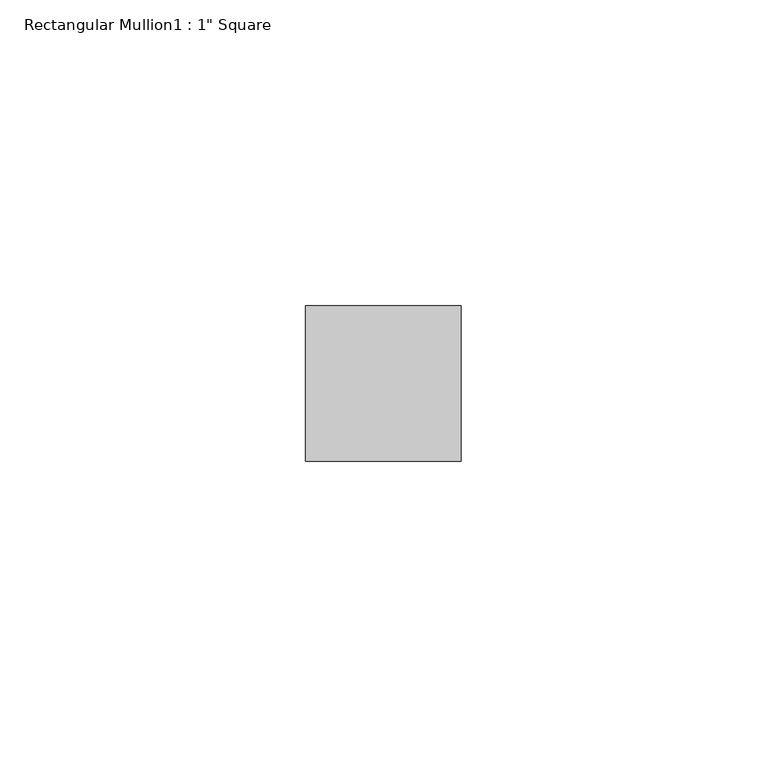
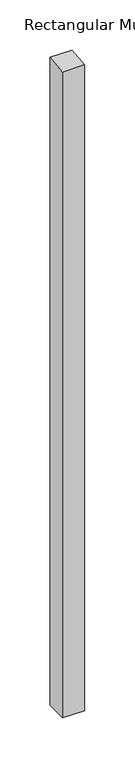
"""IFC4 building model written with IfcOpenShell, lengths in millimetres: member geometry."""

import ifcopenshell
import ifcopenshell.guid

model = None  # the IFC model being written
_history = None  # IfcOwnerHistory: only IFC2X3 demands one
_inside = {}  # id of a spatial element -> (the spatial element, [elements in it])
_under = {}  # id of a project, library or spatial element -> (it, [spatial elements below it])
_declared = {}  # id of a project -> (the project, [libraries it declares])
_typed = {}  # id of a type object -> (the type object, [elements of that type])
_made_of = {}  # id of a material, layer set ... -> (it, [elements and type objects made of it])


def new_model(schema):
    """Start an empty IFC model of exactly this schema.

    Asked for "IFC4X3", IfcOpenShell would pick the latest addendum, in which some entities
    have other attributes; the version numbers below select the first issue.
    IFC2X3 requires an IfcOwnerHistory on every rooted entity: one is made here for all.
    """
    global model, _history
    if schema == "IFC4X3":
        model = ifcopenshell.file(schema_version=(4, 3, 0, 0))
    else:
        model = ifcopenshell.file(schema=schema)
    _inside.clear()
    _under.clear()
    _declared.clear()
    _typed.clear()
    _made_of.clear()
    _history = None
    if model.schema == "IFC2X3":
        org = make("IfcOrganization", Name="unknown")
        user = make(
            "IfcPersonAndOrganization",
            ThePerson=make("IfcPerson", FamilyName="unknown"),
            TheOrganization=org,
        )
        app = make(
            "IfcApplication",
            ApplicationDeveloper=org,
            Version="unknown",
            ApplicationFullName="unknown",
            ApplicationIdentifier="unknown",
        )
        _history = make(
            "IfcOwnerHistory",
            OwningUser=user,
            OwningApplication=app,
            ChangeAction="ADDED",
            CreationDate=0,
        )
    return model


def make(cls, **values):
    """One entity of the class cls with the attributes given. An attribute that is None is left unset."""
    return model.create_entity(
        cls, **{name: value for name, value in values.items() if value is not None}
    )


def rooted(cls, **values):
    """An entity with a GlobalId (a new one), such as an element, a storey or a relation."""
    return make(cls, GlobalId=ifcopenshell.guid.new(), OwnerHistory=_history, **values)


def si_unit(unit_type, name, prefix=None):
    """IfcSIUnit, for example si_unit("LENGTHUNIT", "METRE", prefix="MILLI")."""
    return make("IfcSIUnit", UnitType=unit_type, Prefix=prefix, Name=name)


def assignment(units):
    """IfcUnitAssignment: the units of a project."""
    return None if units is None else make("IfcUnitAssignment", Units=units)


def point(xyz):
    """IfcCartesianPoint."""
    return None if xyz is None else make("IfcCartesianPoint", Coordinates=xyz)


def direction(xyz):
    """IfcDirection."""
    return None if xyz is None else make("IfcDirection", DirectionRatios=xyz)


def frame(location, z_axis=None, x_axis=None):
    """IfcAxis2Placement3D, a coordinate frame: its origin and axes. An axis left out is left unset."""
    return make(
        "IfcAxis2Placement3D",
        Location=point(location),
        Axis=direction(z_axis),
        RefDirection=direction(x_axis),
    )


def origin():
    """The frame at (0, 0, 0) with its axes left unset."""
    return frame((0.0, 0.0, 0.0))


def place(relative_to, where):
    """IfcLocalPlacement: puts the frame where relative to a parent placement (None: the world)."""
    return make(
        "IfcLocalPlacement", PlacementRelTo=relative_to, RelativePlacement=where
    )


def context(
    kind, dimensions, precision=None, world=None, true_north=None, identifier=None
):
    """IfcGeometricRepresentationContext, for example the 3D "Model" context."""
    return make(
        "IfcGeometricRepresentationContext",
        ContextIdentifier=identifier,
        ContextType=kind,
        CoordinateSpaceDimension=dimensions,
        Precision=precision,
        WorldCoordinateSystem=world,
        TrueNorth=true_north,
    )


def project(units=None, contexts=None):
    """IfcProject with its units and contexts."""
    return rooted(
        "IfcProject",
        Name="project",
        RepresentationContexts=contexts,
        UnitsInContext=assignment(units),
    )


def spatial(cls, under=None, at=None, **own):
    """A site, building, storey or space (cls), placed at a placement, below another one or the project."""
    s = rooted(cls, ObjectPlacement=at, **own)
    if under is not None:
        _under.setdefault(under.id(), (under, []))[1].append(s)
    return s


def polyline(points):
    """IfcPolyline through the points."""
    return make("IfcPolyline", Points=[point(p) for p in points])


def outline(outer, holes=None, kind="AREA"):
    """IfcArbitraryClosedProfileDef: a profile drawn as a closed curve; with holes, ...WithVoids."""
    if holes is None:
        return make("IfcArbitraryClosedProfileDef", ProfileType=kind, OuterCurve=outer)
    return make(
        "IfcArbitraryProfileDefWithVoids",
        ProfileType=kind,
        OuterCurve=outer,
        InnerCurves=holes,
    )


def extrude(swept, where, along, depth):
    """IfcExtrudedAreaSolid: the profile swept, set in the frame where, extruded along a direction by depth."""
    return make(
        "IfcExtrudedAreaSolid",
        SweptArea=swept,
        Position=where,
        ExtrudedDirection=direction(along),
        Depth=depth,
    )


def shape(context_of_items, identifier, shape_type, items):
    """IfcShapeRepresentation: the items that make up one representation, for example the "Body"."""
    return make(
        "IfcShapeRepresentation",
        ContextOfItems=context_of_items,
        RepresentationIdentifier=identifier,
        RepresentationType=shape_type,
        Items=items,
    )


def source(mapping_origin, context_of_items, identifier, shape_type, items):
    """IfcRepresentationMap: a shape defined once, which mapped items show again and again."""
    return make(
        "IfcRepresentationMap",
        MappingOrigin=mapping_origin,
        MappedRepresentation=shape(context_of_items, identifier, shape_type, items),
    )


def transform(
    local_origin,
    x_axis=None,
    y_axis=None,
    z_axis=None,
    scale=None,
    scale2=None,
    scale3=None,
    uniform=True,
):
    """IfcCartesianTransformationOperator3D, or its non-uniform kind. x_axis, y_axis, z_axis: its Axis1, 2, 3."""
    if uniform:
        return make(
            "IfcCartesianTransformationOperator3D",
            Axis1=direction(x_axis),
            Axis2=direction(y_axis),
            LocalOrigin=point(local_origin),
            Scale=scale,
            Axis3=direction(z_axis),
        )
    return make(
        "IfcCartesianTransformationOperator3DnonUniform",
        Axis1=direction(x_axis),
        Axis2=direction(y_axis),
        LocalOrigin=point(local_origin),
        Scale=scale,
        Axis3=direction(z_axis),
        Scale2=scale2,
        Scale3=scale3,
    )


def mapped(mapping_source, mapping_target):
    """IfcMappedItem: shows the shape of a source again, moved by a transform."""
    return make(
        "IfcMappedItem", MappingSource=mapping_source, MappingTarget=mapping_target
    )


def made_of(thing, what):
    """Note that an element or type object is made of a material, layer set ...; save() writes the relation."""
    if what is not None:
        _made_of.setdefault(what.id(), (what, []))[1].append(thing)
    return thing


def element(
    cls,
    number,
    at=None,
    inside=None,
    cuts=None,
    type_object=None,
    material=None,
    context=None,
    identifier="Body",
    shape_type=None,
    held_by="IfcProductDefinitionShape",
    body=None,
    shapes=None,
    **own,
):
    """One element of the class cls, such as IfcWall. Its Tag is "e" and its number.

    at: its placement. inside: the storey or other place that contains it. cuts: it is an
    opening in that element (IfcRelVoidsElement). A single representation is given by context,
    identifier, shape_type and body (its items); several are given by shapes. held_by: the class
    of the entity that holds the representations. save() writes the other relations.
    """
    e = rooted(cls, Tag="e%d" % number, ObjectPlacement=at, **own)
    if body is not None:
        shapes = [shape(context, identifier, shape_type, body)]
    if shapes is not None:
        e.Representation = make(held_by, Representations=shapes)
    if inside is not None:
        _inside.setdefault(inside.id(), (inside, []))[1].append(e)
    if cuts is not None:
        rooted(
            "IfcRelVoidsElement", RelatingBuildingElement=cuts, RelatedOpeningElement=e
        )
    if type_object is not None:
        _typed.setdefault(type_object.id(), (type_object, []))[1].append(e)
    return made_of(e, material)


def aggregate(whole, parts):
    """IfcRelAggregates: a whole, such as a stair, and the parts it consists of."""
    return rooted("IfcRelAggregates", RelatingObject=whole, RelatedObjects=parts)


def save(model, path):
    """Write the relations noted so far, then the file.

    IfcRelAggregates (storeys below a building ...), IfcRelContainedInSpatialStructure (elements
    in a storey), IfcRelDefinesByType, IfcRelAssociatesMaterial and IfcRelDeclares: one each for
    every whole, place, type object, material and project.
    """
    for whole, parts in _under.values():
        aggregate(whole, parts)
    for where, things in _inside.values():
        rooted(
            "IfcRelContainedInSpatialStructure",
            RelatedElements=things,
            RelatingStructure=where,
        )
    for kind, things in _typed.values():
        rooted("IfcRelDefinesByType", RelatedObjects=things, RelatingType=kind)
    for what, things in _made_of.values():
        rooted("IfcRelAssociatesMaterial", RelatedObjects=things, RelatingMaterial=what)
    for by, libraries in _declared.values():
        rooted("IfcRelDeclares", RelatingContext=by, RelatedDefinitions=libraries)
    model.write(path)


def member_382b1cd2(model_context):
    return source(origin(), model_context, "Body", "SweptSolid", [
        extrude(outline(polyline([(-44.45, -4.2341647), (-19.05, -1.814642), (-19.05, -790.0272395), (-44.45, -790.0272395), (-44.45, -4.2341647)])), frame((-25.4, 0.0, 0.0), z_axis=(1.0, 0.0, 0.0), x_axis=(0.0, 1.0, 0.0)), (0.0, 0.0, 1.0), 25.4),
    ])


if __name__ == "__main__":
    model = new_model("IFC4")
    model_context = context("Model", 3, world=origin())
    ifc_project = project(units=[si_unit("LENGTHUNIT", "METRE", prefix="MILLI")], contexts=[model_context])
    site = spatial("IfcSite", under=ifc_project)
    building = spatial("IfcBuilding", under=site)
    placement = place(None, origin())
    member_shape = member_382b1cd2(model_context)
    element("IfcMember", 1, ObjectType="Rectangular Mullion1 : 1\" Square", at=placement, inside=building, context=model_context, shape_type="MappedRepresentation", body=[
        mapped(member_shape, transform((0.0, 0.0, 0.0), x_axis=(1.0, 0.0, 0.0), y_axis=(0.0, 1.0, 0.0), z_axis=(0.0, 0.0, 1.0))),
    ])
    save(model, "model.ifc")

# Revit data of these elements
# Type "Rectangular Mullion1 : 1\" Square"
#   built-in parameter 1007351 = 0.104167 (stored number, unit not read)
#   built-in parameter 1007304 = 0.0833333 (stored number, unit not read)
#   built-in parameter 1007301 = 0.0416667 (stored number, unit not read)
#   built-in parameter 1007300 = 0.0416667 (stored number, unit not read)
